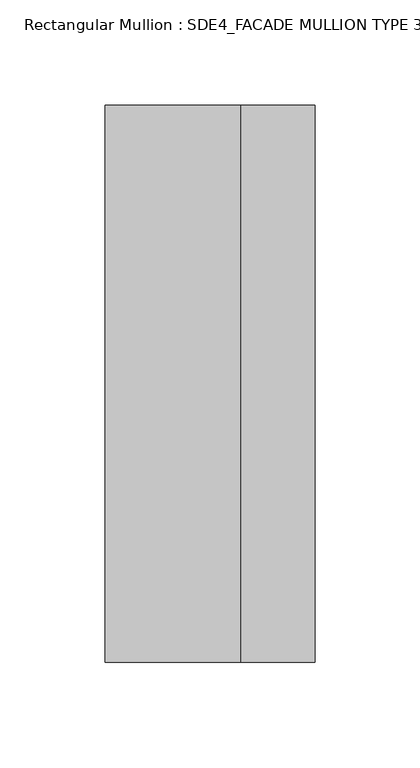
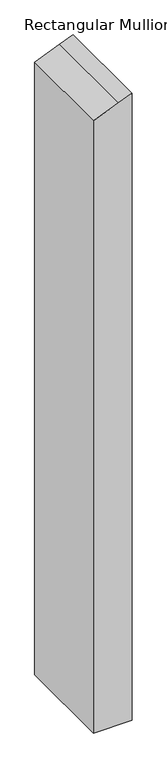
"""IFC4 building model written with IfcOpenShell, lengths in millimetres: member geometry, Rectangular Mullion : SDE4_FACADE MULLION TYPE 3."""

import ifcopenshell
import ifcopenshell.guid

model = None  # the IFC model being written
_history = None  # IfcOwnerHistory: only IFC2X3 demands one
_inside = {}  # id of a spatial element -> (the spatial element, [elements in it])
_under = {}  # id of a project, library or spatial element -> (it, [spatial elements below it])
_declared = {}  # id of a project -> (the project, [libraries it declares])
_typed = {}  # id of a type object -> (the type object, [elements of that type])
_made_of = {}  # id of a material, layer set ... -> (it, [elements and type objects made of it])


def new_model(schema):
    """Start an empty IFC model of exactly this schema.

    Asked for "IFC4X3", IfcOpenShell would pick the latest addendum, in which some entities
    have other attributes; the version numbers below select the first issue.
    IFC2X3 requires an IfcOwnerHistory on every rooted entity: one is made here for all.
    """
    global model, _history
    if schema == "IFC4X3":
        model = ifcopenshell.file(schema_version=(4, 3, 0, 0))
    else:
        model = ifcopenshell.file(schema=schema)
    _inside.clear()
    _under.clear()
    _declared.clear()
    _typed.clear()
    _made_of.clear()
    _history = None
    if model.schema == "IFC2X3":
        org = make("IfcOrganization", Name="unknown")
        user = make(
            "IfcPersonAndOrganization",
            ThePerson=make("IfcPerson", FamilyName="unknown"),
            TheOrganization=org,
        )
        app = make(
            "IfcApplication",
            ApplicationDeveloper=org,
            Version="unknown",
            ApplicationFullName="unknown",
            ApplicationIdentifier="unknown",
        )
        _history = make(
            "IfcOwnerHistory",
            OwningUser=user,
            OwningApplication=app,
            ChangeAction="ADDED",
            CreationDate=0,
        )
    return model


def make(cls, **values):
    """One entity of the class cls with the attributes given. An attribute that is None is left unset."""
    return model.create_entity(
        cls, **{name: value for name, value in values.items() if value is not None}
    )


def rooted(cls, **values):
    """An entity with a GlobalId (a new one), such as an element, a storey or a relation."""
    return make(cls, GlobalId=ifcopenshell.guid.new(), OwnerHistory=_history, **values)


def si_unit(unit_type, name, prefix=None):
    """IfcSIUnit, for example si_unit("LENGTHUNIT", "METRE", prefix="MILLI")."""
    return make("IfcSIUnit", UnitType=unit_type, Prefix=prefix, Name=name)


def assignment(units):
    """IfcUnitAssignment: the units of a project."""
    return None if units is None else make("IfcUnitAssignment", Units=units)


def point(xyz):
    """IfcCartesianPoint."""
    return None if xyz is None else make("IfcCartesianPoint", Coordinates=xyz)


def direction(xyz):
    """IfcDirection."""
    return None if xyz is None else make("IfcDirection", DirectionRatios=xyz)


def frame(location, z_axis=None, x_axis=None):
    """IfcAxis2Placement3D, a coordinate frame: its origin and axes. An axis left out is left unset."""
    return make(
        "IfcAxis2Placement3D",
        Location=point(location),
        Axis=direction(z_axis),
        RefDirection=direction(x_axis),
    )


def origin():
    """The frame at (0, 0, 0) with its axes left unset."""
    return frame((0.0, 0.0, 0.0))


def place(relative_to, where):
    """IfcLocalPlacement: puts the frame where relative to a parent placement (None: the world)."""
    return make(
        "IfcLocalPlacement", PlacementRelTo=relative_to, RelativePlacement=where
    )


def context(
    kind, dimensions, precision=None, world=None, true_north=None, identifier=None
):
    """IfcGeometricRepresentationContext, for example the 3D "Model" context."""
    return make(
        "IfcGeometricRepresentationContext",
        ContextIdentifier=identifier,
        ContextType=kind,
        CoordinateSpaceDimension=dimensions,
        Precision=precision,
        WorldCoordinateSystem=world,
        TrueNorth=true_north,
    )


def project(units=None, contexts=None):
    """IfcProject with its units and contexts."""
    return rooted(
        "IfcProject",
        Name="project",
        RepresentationContexts=contexts,
        UnitsInContext=assignment(units),
    )


def spatial(cls, under=None, at=None, **own):
    """A site, building, storey or space (cls), placed at a placement, below another one or the project."""
    s = rooted(cls, ObjectPlacement=at, **own)
    if under is not None:
        _under.setdefault(under.id(), (under, []))[1].append(s)
    return s


def polyline(points):
    """IfcPolyline through the points."""
    return make("IfcPolyline", Points=[point(p) for p in points])


def outline(outer, holes=None, kind="AREA"):
    """IfcArbitraryClosedProfileDef: a profile drawn as a closed curve; with holes, ...WithVoids."""
    if holes is None:
        return make("IfcArbitraryClosedProfileDef", ProfileType=kind, OuterCurve=outer)
    return make(
        "IfcArbitraryProfileDefWithVoids",
        ProfileType=kind,
        OuterCurve=outer,
        InnerCurves=holes,
    )


def extrude(swept, where, along, depth):
    """IfcExtrudedAreaSolid: the profile swept, set in the frame where, extruded along a direction by depth."""
    return make(
        "IfcExtrudedAreaSolid",
        SweptArea=swept,
        Position=where,
        ExtrudedDirection=direction(along),
        Depth=depth,
    )


def shape(context_of_items, identifier, shape_type, items):
    """IfcShapeRepresentation: the items that make up one representation, for example the "Body"."""
    return make(
        "IfcShapeRepresentation",
        ContextOfItems=context_of_items,
        RepresentationIdentifier=identifier,
        RepresentationType=shape_type,
        Items=items,
    )


def source(mapping_origin, context_of_items, identifier, shape_type, items):
    """IfcRepresentationMap: a shape defined once, which mapped items show again and again."""
    return make(
        "IfcRepresentationMap",
        MappingOrigin=mapping_origin,
        MappedRepresentation=shape(context_of_items, identifier, shape_type, items),
    )


def transform(
    local_origin,
    x_axis=None,
    y_axis=None,
    z_axis=None,
    scale=None,
    scale2=None,
    scale3=None,
    uniform=True,
):
    """IfcCartesianTransformationOperator3D, or its non-uniform kind. x_axis, y_axis, z_axis: its Axis1, 2, 3."""
    if uniform:
        return make(
            "IfcCartesianTransformationOperator3D",
            Axis1=direction(x_axis),
            Axis2=direction(y_axis),
            LocalOrigin=point(local_origin),
            Scale=scale,
            Axis3=direction(z_axis),
        )
    return make(
        "IfcCartesianTransformationOperator3DnonUniform",
        Axis1=direction(x_axis),
        Axis2=direction(y_axis),
        LocalOrigin=point(local_origin),
        Scale=scale,
        Axis3=direction(z_axis),
        Scale2=scale2,
        Scale3=scale3,
    )


def mapped(mapping_source, mapping_target):
    """IfcMappedItem: shows the shape of a source again, moved by a transform."""
    return make(
        "IfcMappedItem", MappingSource=mapping_source, MappingTarget=mapping_target
    )


def made_of(thing, what):
    """Note that an element or type object is made of a material, layer set ...; save() writes the relation."""
    if what is not None:
        _made_of.setdefault(what.id(), (what, []))[1].append(thing)
    return thing


def element(
    cls,
    number,
    at=None,
    inside=None,
    cuts=None,
    type_object=None,
    material=None,
    context=None,
    identifier="Body",
    shape_type=None,
    held_by="IfcProductDefinitionShape",
    body=None,
    shapes=None,
    **own,
):
    """One element of the class cls, such as IfcWall. Its Tag is "e" and its number.

    at: its placement. inside: the storey or other place that contains it. cuts: it is an
    opening in that element (IfcRelVoidsElement). A single representation is given by context,
    identifier, shape_type and body (its items); several are given by shapes. held_by: the class
    of the entity that holds the representations. save() writes the other relations.
    """
    e = rooted(cls, Tag="e%d" % number, ObjectPlacement=at, **own)
    if body is not None:
        shapes = [shape(context, identifier, shape_type, body)]
    if shapes is not None:
        e.Representation = make(held_by, Representations=shapes)
    if inside is not None:
        _inside.setdefault(inside.id(), (inside, []))[1].append(e)
    if cuts is not None:
        rooted(
            "IfcRelVoidsElement", RelatingBuildingElement=cuts, RelatedOpeningElement=e
        )
    if type_object is not None:
        _typed.setdefault(type_object.id(), (type_object, []))[1].append(e)
    return made_of(e, material)


def aggregate(whole, parts):
    """IfcRelAggregates: a whole, such as a stair, and the parts it consists of."""
    return rooted("IfcRelAggregates", RelatingObject=whole, RelatedObjects=parts)


def save(model, path):
    """Write the relations noted so far, then the file.

    IfcRelAggregates (storeys below a building ...), IfcRelContainedInSpatialStructure (elements
    in a storey), IfcRelDefinesByType, IfcRelAssociatesMaterial and IfcRelDeclares: one each for
    every whole, place, type object, material and project.
    """
    for whole, parts in _under.values():
        aggregate(whole, parts)
    for where, things in _inside.values():
        rooted(
            "IfcRelContainedInSpatialStructure",
            RelatedElements=things,
            RelatingStructure=where,
        )
    for kind, things in _typed.values():
        rooted("IfcRelDefinesByType", RelatedObjects=things, RelatingType=kind)
    for what, things in _made_of.values():
        rooted("IfcRelAssociatesMaterial", RelatedObjects=things, RelatingMaterial=what)
    for by, libraries in _declared.values():
        rooted("IfcRelDeclares", RelatingContext=by, RelatedDefinitions=libraries)
    model.write(path)


def rectangular_mullion_sde4_facade_mullion_type_3_c874baf2(model_context):
    return source(origin(), model_context, "Body", "SweptSolid", [
        extrude(outline(polyline([(-23.0813185, 50.0), (-37.1390676, 14.8556271), (-63.0813185, -50.0), (-1747.974544, -50.0), (-1747.974544, 50.0), (-23.0813185, 50.0)])), frame((0.0, -132.5, 0.0), z_axis=(0.0, 1.0, 0.0), x_axis=(0.0, 0.0, 1.0)), (0.0, 0.0, 1.0), 265.0),
    ])


if __name__ == "__main__":
    model = new_model("IFC4")
    model_context = context("Model", 3, world=origin())
    ifc_project = project(units=[si_unit("LENGTHUNIT", "METRE", prefix="MILLI")], contexts=[model_context])
    site = spatial("IfcSite", under=ifc_project)
    building = spatial("IfcBuilding", under=site)
    placement = place(None, origin())
    rectangular_mullion_sde4_facade_mullion_type_3_shape = rectangular_mullion_sde4_facade_mullion_type_3_c874baf2(model_context)
    element("IfcMember", 1, ObjectType="Rectangular Mullion : SDE4_FACADE MULLION TYPE 3", at=placement, inside=building, context=model_context, shape_type="MappedRepresentation", body=[
        mapped(rectangular_mullion_sde4_facade_mullion_type_3_shape, transform((0.0, 0.0, 0.0), x_axis=(1.0, 0.0, 0.0), y_axis=(0.0, 1.0, 0.0), z_axis=(0.0, 0.0, 1.0))),
    ])
    save(model, "model.ifc")

# Revit data of these elements
# Type "Rectangular Mullion : SDE4_FACADE MULLION TYPE 3"
#   built-in parameter 1007322 = 0.869423 (stored number, unit not read)
#   built-in parameter 1007321 = 0.164042 (stored number, unit not read)
#   built-in parameter 1007320 = 0.164042 (stored number, unit not read)
